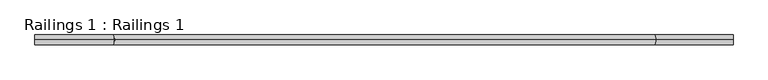
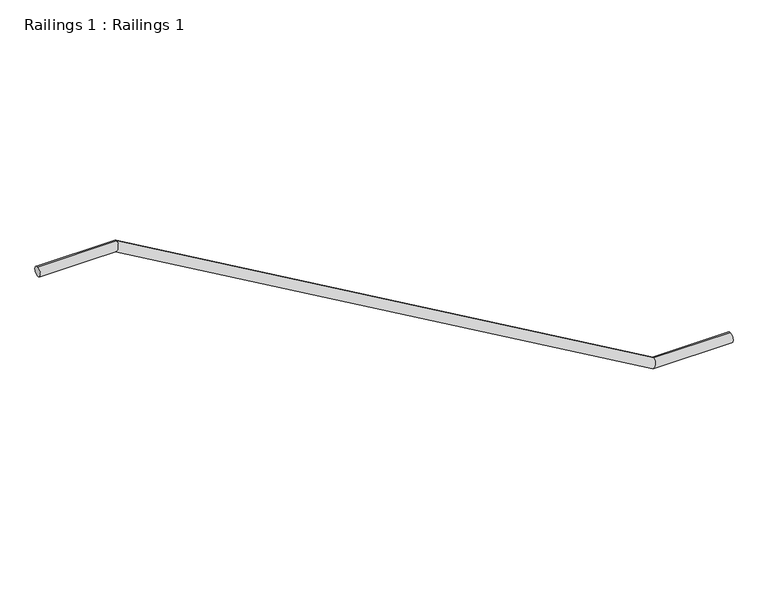
"""IFC4 building model written with IfcOpenShell, lengths in millimetres: railing geometry, Railings 1 : Railings 1."""

from ifc_helpers import new_model, si_unit, frame, origin, place, context, project, spatial, circle_curve, ellipse_curve, source, transform, mapped, element, save
from ifc_brep_helpers import plane_surface, cylinder_surface, advanced_brep


def railings_1_railings_1_3b98a546(model_context):
    return source(origin(), model_context, "Body", "AdvancedBrep", [
        advanced_brep(
        [(31978.7088966, 25437.1656612, 264889.3189609), (31978.7088966, 25437.1656612, 264851.2189609), (31679.0363282, 25437.1656612, 264889.3189609), (31668.7814649, 25437.1656612, 264851.2189609), (29570.8363282, 25437.1656612, 266112.8278895), (29560.5814649, 25437.1656612, 266074.7278895), (29260.9088966, 25437.1656612, 266112.8278895), (29260.9088966, 25437.1656612, 266074.7278895)],
        [
            (0, 1, circle_curve(frame((31978.7088966, 25437.1656612, 264870.2689609), z_axis=(1.0, 0.0, 0.0), x_axis=(0.0, 0.0, -1.0)), 19.05)),
            (1, 0, circle_curve(frame((31978.7088966, 25437.1656612, 264870.2689609), z_axis=(1.0, 0.0, 0.0), x_axis=(0.0, 0.0, -1.0)), 19.05)),
            (0, 2),
            (2, 3, ellipse_curve(frame((31673.9088966, 25437.1656612, 264870.2689609), z_axis=(0.9656337553070279, 0.0, -0.2599066190223847), x_axis=(0.25990661902238477, 0.0, 0.965633755307028)), 19.7279765, 19.05)),
            (3, 1),
            (3, 2, ellipse_curve(frame((31673.9088966, 25437.1656612, 264870.2689609), z_axis=(0.9656337553070279, 0.0, -0.2599066190223847), x_axis=(0.25990661902238477, 0.0, 0.965633755307028)), 19.7279765, 19.05)),
            (2, 4),
            (4, 5, ellipse_curve(frame((29565.7088966, 25437.1656612, 266093.7778895), z_axis=(0.9656337553070279, 0.0, -0.2599066190223847), x_axis=(-0.25990661902238477, 0.0, -0.965633755307028)), 19.7279765, 19.05)),
            (5, 3),
            (5, 4, ellipse_curve(frame((29565.7088966, 25437.1656612, 266093.7778895), z_axis=(0.9656337553070279, 0.0, -0.2599066190223847), x_axis=(-0.25990661902238477, 0.0, -0.965633755307028)), 19.7279765, 19.05)),
            (6, 7, circle_curve(frame((29260.9088966, 25437.1656612, 266093.7778895), z_axis=(-1.0, 0.0, 0.0), x_axis=(0.0, 0.0, -1.0)), 19.05)),
            (7, 6, circle_curve(frame((29260.9088966, 25437.1656612, 266093.7778895), z_axis=(-1.0, 0.0, 0.0), x_axis=(0.0, 0.0, -1.0)), 19.05)),
            (4, 6),
            (7, 5),
        ],
        [
            plane_surface(frame((31978.7088966, 25418.1156612, 264870.2689609), z_axis=(1.0, 0.0, 0.0), x_axis=(0.0, -1.0, 0.0))),
            cylinder_surface(frame((31978.7088966, 25437.1656612, 264870.2689609), z_axis=(1.0, 0.0, 0.0), x_axis=(0.0, 0.0, -1.0)), 19.05),
            cylinder_surface(frame((31673.9088966, 25437.1656612, 264870.2689609), z_axis=(0.864897098776706, 0.0, -0.5019492091114767), x_axis=(-0.5019492091114767, 0.0, -0.864897098776706)), 19.05),
            plane_surface(frame((29260.9088966, 25418.1156612, 266093.7778895), z_axis=(-1.0, 0.0, 0.0), x_axis=(0.0, -1.0, 0.0))),
            cylinder_surface(frame((29565.7088966, 25437.1656612, 266093.7778895), z_axis=(1.0, 0.0, 0.0), x_axis=(0.0, 0.0, -1.0)), 19.05),
        ],
        [
            (0, [[1, 2]]),
            (1, [[-1, 3, 4, 5]]),
            (1, [[-2, -5, 6, -3]]),
            (2, [[-4, 7, 8, 9]]),
            (2, [[-6, -9, 10, -7]]),
            (3, [[11, 12]]),
            (4, [[-8, 13, -12, 14]]),
            (4, [[-10, -14, -11, -13]]),
        ],
    ),
    ])


if __name__ == "__main__":
    model = new_model("IFC4")
    model_context = context("Model", 3, world=origin())
    ifc_project = project(units=[si_unit("LENGTHUNIT", "METRE", prefix="MILLI")], contexts=[model_context])
    site = spatial("IfcSite", under=ifc_project)
    building = spatial("IfcBuilding", under=site)
    placement = place(None, origin())
    railings_1_railings_1_shape = railings_1_railings_1_3b98a546(model_context)
    element("IfcRailing", 1, ObjectType="Railings 1 : Railings 1", at=placement, inside=building, context=model_context, shape_type="MappedRepresentation", body=[
        mapped(railings_1_railings_1_shape, transform((0.0, 0.0, 0.0), x_axis=(1.0, 0.0, 0.0), y_axis=(0.0, 1.0, 0.0), z_axis=(0.0, 0.0, 1.0))),
    ])
    save(model, "model.ifc")

# Revit data of these elements
# Element 1 (IfcRailing, "Railings 1 : Railings 1")
#   Materials on its faces: "ALUM. RAILING"
# Materials
#   "ALUM. RAILING": class "Generic", colour RGB 255 255 255, transparency 0, Cost = 0
